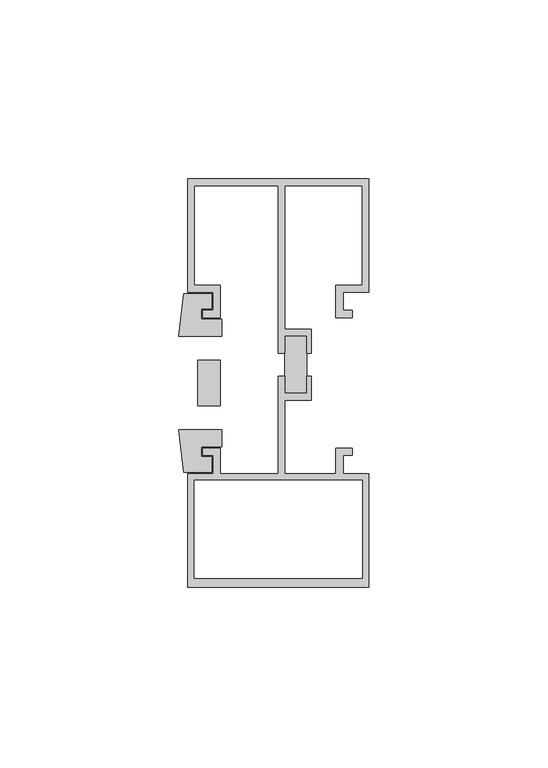
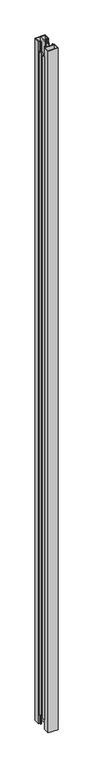
"""IFC4 building model written with IfcOpenShell, lengths in millimetres: proxy geometry, Generic Models 3:Generic Models 1:5:Generic Models 1:5 : Generic Models 3:Generic Models 1:300625:345888:Generic Models 1:5:Generic Models 1:5 : Generic Models 3:Generic Models 1:300625:345888 : Generic Models 3:Generic Models 1:5:Generic Models 1:5 : Generic Models 3:Generic Models 1:300625:345888:2 : Generic Models 3:Generic Models 1:5:Generic Models 1:5 : Generic Models 3:Generic Models 1:300625:345888:Generic Models 1:5:Generic Models 1:5 : Generic Models 3:Generic Models 1:300625:345888 : Generic Models 3:Generic Models 1:5:Generic Models 1:5 : Generic Models 3:Generic Models 1:300625:345888:301574."""

from ifc_helpers import new_model, si_unit, frame, origin, place, context, project, spatial, polyline, outline, extrude, source, transform, mapped, element, save


def generic_models_cbd6f345(model_context):
    return source(origin(), model_context, "Body", "SweptSolid", [
        extrude(outline(polyline([(593708.2535457, -579063.9802804), (593708.2535457, -579047.8688442), (593714.333333, -579047.8688442), (593714.333333, -579063.9802804), (593708.2535457, -579063.9802804)])), frame((0.0, 0.0, 82.9809556), z_axis=(0.0, 0.0, 1.0), x_axis=(1.0, 0.0, 0.0)), (0.0, 0.0, 1.0), 3568.302821),
        extrude(outline(polyline([(593683.8226303, -579067.3663841), (593683.8226303, -579054.6663841), (593690.1661787, -579054.6663841), (593690.1661787, -579067.3663841), (593683.8226303, -579067.3663841)])), frame((0.0, 0.0, 82.9809556), z_axis=(0.0, 0.0, 1.0), x_axis=(1.0, 0.0, 0.0)), (0.0, 0.0, 1.0), 3568.302821),
        extrude(outline(polyline([(593684.8495131, -579078.8588708), (593684.8495131, -579081.704549), (593687.7933729, -579081.704549), (593687.7933729, -579086.0026208), (593679.9536635, -579086.0026208), (593678.4927966, -579074.1048149), (593690.5630537, -579074.1048149), (593690.5630537, -579078.8588708), (593684.8495131, -579078.8588708)])), frame((0.0, 0.0, 82.9809556), z_axis=(0.0, 0.0, 1.0), x_axis=(1.0, 0.0, 0.0)), (0.0, 0.0, 1.0), 3568.302821),
        extrude(outline(polyline([(593679.9536635, -579036.0301474), (593687.7933729, -579036.0301474), (593687.7933729, -579040.3282192), (593684.8495131, -579040.3282192), (593684.8495131, -579043.1738974), (593690.5630537, -579043.1738974), (593690.5630537, -579047.9279532), (593678.4927966, -579047.9279532), (593679.9536635, -579036.0301474)])), frame((0.0, 0.0, 82.9809556), z_axis=(0.0, 0.0, 1.0), x_axis=(1.0, 0.0, 0.0)), (0.0, 0.0, 1.0), 3568.2690444),
        extrude(outline(polyline([(593731.7367239, -579118.1663841), (593680.9705005, -579118.1663841), (593680.9705005, -579086.3994958), (593688.1902479, -579086.3994958), (593688.1902479, -579081.307674), (593685.2463881, -579081.307674), (593685.2463881, -579079.2557458), (593690.1661787, -579079.2557458), (593690.1661787, -579086.3994958), (593706.3536122, -579086.3994958), (593706.3536122, -579059.1164506), (593708.2535457, -579059.1164506), (593708.2535457, -579063.9802804), (593714.333333, -579063.9802804), (593714.333333, -579059.1164506), (593715.6252878, -579059.1164506), (593715.6252878, -579065.8802139), (593708.2535457, -579065.8802139), (593708.2535457, -579086.3994958), (593722.4650484, -579086.3994958), (593722.4650484, -579079.2557458), (593727.036208, -579079.2557458), (593727.036208, -579081.307674), (593724.5169766, -579081.307674), (593724.5169766, -579086.3994958), (593731.7367239, -579086.3994958), (593731.7367239, -579118.1663841)]), holes=[polyline([(593682.870434, -579088.2994293), (593682.870434, -579115.6584719), (593729.8367904, -579115.6584719), (593729.8367904, -579088.2994293), (593682.870434, -579088.2994293)])]), frame((0.0, 0.0, 30.7803608), z_axis=(0.0, 0.0, 1.0), x_axis=(1.0, 0.0, 0.0)), (0.0, 0.0, 1.0), 3671.2696392),
        extrude(outline(polyline([(593685.2463881, -579040.7250942), (593688.1902479, -579040.7250942), (593688.1902479, -579035.6332724), (593680.9705005, -579035.6332724), (593680.9705005, -579003.8663841), (593731.7367239, -579003.8663841), (593731.7367239, -579035.6332724), (593724.5169766, -579035.6332724), (593724.5169766, -579040.7250942), (593727.036208, -579040.7250942), (593727.036208, -579042.7770224), (593722.4650484, -579042.7770224), (593722.4650484, -579033.7333389), (593729.8145113, -579033.7333389), (593729.8145113, -579005.8423149), (593708.2535457, -579005.8423149), (593708.2535457, -579045.9689107), (593715.6252878, -579045.9689107), (593715.6252878, -579052.732674), (593714.333333, -579052.732674), (593714.333333, -579047.8688442), (593708.2535457, -579047.8688442), (593708.2535457, -579052.732674), (593706.3536122, -579052.732674), (593706.3536122, -579005.8423149), (593682.8802996, -579005.8423149), (593682.8802996, -579033.7333389), (593690.1661787, -579033.7333389), (593690.1661787, -579042.7770224), (593685.2463881, -579042.7770224), (593685.2463881, -579040.7250942)])), frame((0.0, 0.0, 30.7803608), z_axis=(0.0, 0.0, 1.0), x_axis=(1.0, 0.0, 0.0)), (0.0, 0.0, 1.0), 3671.2696392),
    ])


if __name__ == "__main__":
    model = new_model("IFC4")
    model_context = context("Model", 3, world=origin())
    ifc_project = project(units=[si_unit("LENGTHUNIT", "METRE", prefix="MILLI")], contexts=[model_context])
    site = spatial("IfcSite", under=ifc_project)
    building = spatial("IfcBuilding", under=site)
    placement = place(None, origin())
    generic_models_shape = generic_models_cbd6f345(model_context)
    element("IfcBuildingElementProxy", 1, Name="Generic Models 3:Generic Models 1:5:Generic Models 1:5 : Generic Models 3:Generic Models 1:300625:345888:Generic Models 1:5:Generic Models 1:5 : Generic Models 3:Generic Models 1:300625:345888 : Generic Models 3:Generic Models 1:5:Generic Models 1:5 : Generic Models 3:Generic Models 1:300625:345888:2 : Generic Models 3:Generic Models 1:5:Generic Models 1:5 : Generic Models 3:Generic Models 1:300625:345888:Generic Models 1:5:Generic Models 1:5 : Generic Models 3:Generic Models 1:300625:345888 : Generic Models 3:Generic Models 1:5:Generic Models 1:5 : Generic Models 3:Generic Models 1:300625:345888:301574", ObjectType="Generic Models 3:Generic Models 1:5:Generic Models 1:5 : Generic Models 3:Generic Models 1:300625:345888:Generic Models 1:5:Generic Models 1:5 : Generic Models 3:Generic Models 1:300625:345888 : Generic Models 3:Generic Models 1:5:Generic Models 1:5 : Generic Models 3:Generic Models 1:300625:345888:2 : Generic Models 3:Generic Models 1:5:Generic Models 1:5 : Generic Models 3:Generic Models 1:300625:345888:Generic Models 1:5:Generic Models 1:5 : Generic Models 3:Generic Models 1:300625:345888 : Generic Models 3:Generic Models 1:5:Generic Models 1:5 : Generic Models 3:Generic Models 1:300625:345888:301574", at=placement, inside=building, context=model_context, shape_type="MappedRepresentation", body=[
        mapped(generic_models_shape, transform((0.0, 0.0, 0.0), x_axis=(1.0, 0.0, 0.0), y_axis=(0.0, 1.0, 0.0), z_axis=(0.0, 0.0, 1.0))),
    ])
    save(model, "model.ifc")

# Revit data of these elements
# Type "Generic Models 3:Generic Models 1:5:Generic Models 1:5 : Generic Models 3:Generic Models 1:300625:345888:Generic Models 1:5:Generic Models 1:5 : Generic Models 3:Generic Models 1:300625:345888 : Generic Models 3:Generic Models 1:5:Generic Models 1:5 : Generic Models 3:Generic Models 1:300625:345888:2 : Generic Models 3:Generic Models 1:5:Generic Models 1:5 : Generic Models 3:Generic Models 1:300625:345888:Generic Models 1:5:Generic Models 1:5 : Generic Models 3:Generic Models 1:300625:345888 : Generic Models 3:Generic Models 1:5:Generic Models 1:5 : Generic Models 3:Generic Models 1:300625:345888:301574"
#   NameOverride = "Generic Models 3:Generic Models 1:5:Generic Models 1:5 : Generic Models 3:Generic Models 1:300625:345888:Generic Models 1:5:Generic Models 1:5 : Generic Models 3:Generic Models 1:300625:345888 : Generic Models 3:Generic Models 1:5:Generic Models 1:5 : Generic Models 3:Generic Models 1:300625:345888:301574"
#   ObjectTypeOverride = "Generic Models 1:5:Generic Models 1:5 : Generic Models 3:Generic Models 1:300625:345888 : Generic Models 3:Generic Models 1:5:Generic Models 1:5 : Generic Models 3:Generic Models 1:300625:345888"
#   Reference = "Generic Models 1"
#   Tag = "301574"
# Element 1 (IfcBuildingElementProxy, "Generic Models 3:Generic Models 1:5:Generic Models 1:5 : Generic Models 3:Generic Models 1:300625:345888:Generic Models 1:5:Generic Models 1:5 : Generic Models 3:Generic Models 1:300625:345888 : Generic Models 3:Generic Models 1:5:Generic Models 1:5 : Generic Models 3:Generic Models 1:300625:345888:2 : Generic Models 3:Generic Models 1:5:Generic Models 1:5 : Generic Models 3:Generic Models 1:300625:345888:Generic Models 1:5:Generic Models 1:5 : Generic Models 3:Generic Models 1:300625:345888 : Generic Models 3:Generic Models 1:5:Generic Models 1:5 : Generic Models 3:Generic Models 1:300625:345888:301574")
#   Materials on its faces: "THERMAL BROKEN ALUMINUM STOREFRONT"
# Materials
#   "THERMAL BROKEN ALUMINUM STOREFRONT": class "Unassigned", colour RGB 244 244 244, transparency 0, Cost = 0
